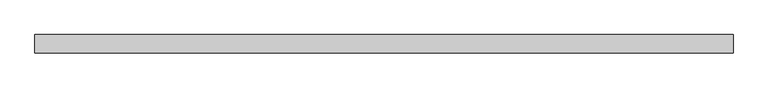
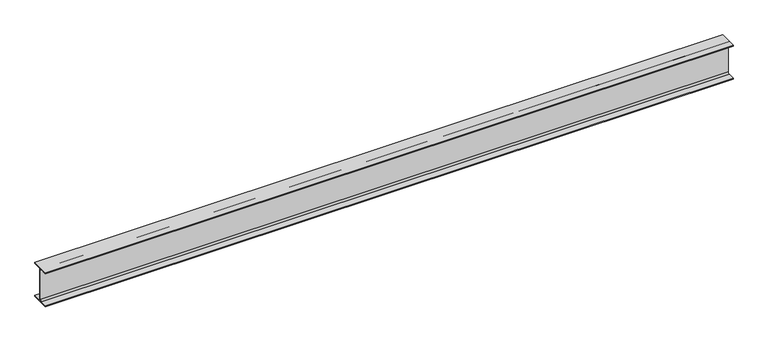
"""IFC4 building model written with IfcOpenShell, lengths in millimetres: beam geometry, Steel Framing_H_KS : H_SB_AR_S02_H-300x150x6.5x9_SRB3."""

from ifc_helpers import new_model, si_unit, point, frame, frame_2d, origin, place, context, project, spatial, polyline, circle_curve, trimmed, segment, composite_curve, outline, extrude, source, transform, mapped, element, save


def beam_8c59a53e(model_context):
    return source(origin(), model_context, "Body", "SweptSolid", [
        extrude(outline(composite_curve([segment(polyline([(75.0, -141.0), (75.0, -150.0), (-75.0, -150.0), (-75.0, -141.0), (-16.25, -141.0)]), True, "CONTINUOUS"), segment(trimmed(circle_curve(frame_2d((-16.25, -128.0)), 13.0), [point((-16.25, -141.0))], [point((-3.25, -128.0))], True, "CARTESIAN"), True, "CONTINUOUS"), segment(polyline([(-3.25, -128.0), (-3.25, 128.0)]), True, "CONTINUOUS"), segment(trimmed(circle_curve(frame_2d((-16.25, 128.0)), 13.0), [point((-3.25, 128.0))], [point((-16.25, 141.0))], True, "CARTESIAN"), True, "CONTINUOUS"), segment(polyline([(-16.25, 141.0), (-75.0, 141.0), (-75.0, 150.0), (75.0, 150.0), (75.0, 141.0), (16.25, 141.0)]), True, "CONTINUOUS"), segment(trimmed(circle_curve(frame_2d((16.25, 128.0)), 13.0), [point((16.25, 141.0))], [point((3.25, 128.0))], True, "CARTESIAN"), True, "CONTINUOUS"), segment(polyline([(3.25, 128.0), (3.25, -128.0)]), True, "CONTINUOUS"), segment(trimmed(circle_curve(frame_2d((16.25, -128.0)), 13.0), [point((3.25, -128.0))], [point((16.25, -141.0))], True, "CARTESIAN"), True, "CONTINUOUS"), segment(polyline([(16.25, -141.0), (75.0, -141.0)]), True, "CONTINUOUS")], self_intersect=False)), frame((-2887.3, 0.0, 0.0), z_axis=(1.0, 0.0, 0.0), x_axis=(0.0, 1.0, 0.0)), (0.0, 0.0, 1.0), 5724.6),
    ])


if __name__ == "__main__":
    model = new_model("IFC4")
    model_context = context("Model", 3, world=origin())
    ifc_project = project(units=[si_unit("LENGTHUNIT", "METRE", prefix="MILLI")], contexts=[model_context])
    site = spatial("IfcSite", under=ifc_project)
    building = spatial("IfcBuilding", under=site)
    placement = place(None, origin())
    beam_shape = beam_8c59a53e(model_context)
    element("IfcBeam", 1, ObjectType="Steel Framing_H_KS : H_SB_AR_S02_H-300x150x6.5x9_SRB3", at=placement, inside=building, context=model_context, shape_type="MappedRepresentation", body=[
        mapped(beam_shape, transform((0.0, 0.0, 0.0), x_axis=(1.0, 0.0, 0.0), y_axis=(0.0, 1.0, 0.0), z_axis=(0.0, 0.0, 1.0))),
    ])
    save(model, "model.ifc")

# Revit data of these elements
# Type "Steel Framing_H_KS : H_SB_AR_S02_H-300x150x6.5x9_SRB3"
#   Type Comments = "MAIN"
#   Type Mark = "SRB3"
#   H_SectionID = "H-300x150x6.5x9"
#   H_Ratio for Additional Steel Plate = 0.2
#   Width = 15.0 cm
#   Web Thickness = 0.65 cm
#   Web Fillet = 1.3 cm
#   Warping Constant = 107000.0 cm⁶
#   Torsional Moment of Inertia = 9.9539 cm⁴
#   Section Area = 46.78 cm²
#   Plastic Modulus weak axis = 105.0 cm³
#   Plastic Modulus strong axis = 542.0 cm³
#   Perimeter = 1.17 m²/m
#   Nominal Weight = 36.70 kgf/m
#   Moment of Inertia weak axis = 508.00 cm⁴
#   Moment of Inertia strong axis = 7210.00 cm⁴
#   Height = 30.0 cm
#   Flange Thickness = 0.9 cm
#   Elastic Modulus weak axis = 67.7 cm³
#   Elastic Modulus strong axis = 481.0 cm³
#   Centroid Vertical = 15.0 cm
#   Centroid Horizontal = 7.5 cm
#   Bolt Spacing = 8.89 cm
#   Length [instance default] = 1500 mm
#   Structural Material [instance default] = Steel, 45-345
#   Section Name Key = ""
#   Assembly Code = ""
# Element 1 (IfcBeam, "Steel Framing_H_KS : H_SB_AR_S02_H-300x150x6.5x9_SRB3")
#   Materials on its faces: "Steel, 45-345"
# Materials
#   "Steel, 45-345": class "Metal", colour RGB 189 187 185, transparency 0, Description = "Steel 345 MPa", Cost = 0
